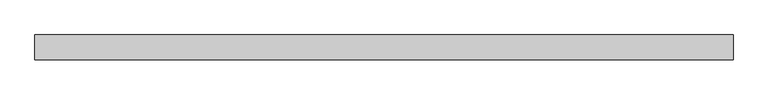
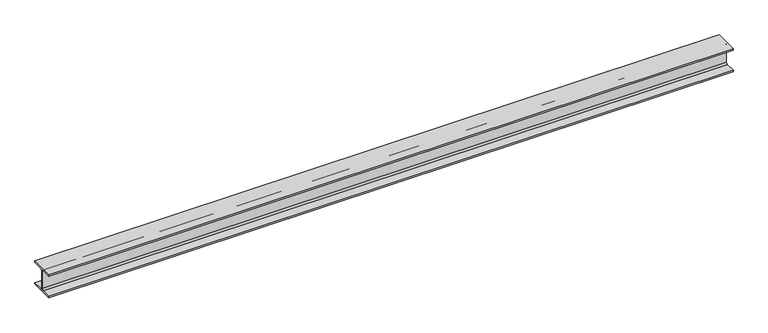
"""IFC4 building model written with IfcOpenShell, lengths in millimetres: beam geometry, 0912_Steel Framing_H-KSD3502 : H_SB_ASB_H-200x200x8x12."""

import ifcopenshell
import ifcopenshell.guid

model = None  # the IFC model being written
_history = None  # IfcOwnerHistory: only IFC2X3 demands one
_inside = {}  # id of a spatial element -> (the spatial element, [elements in it])
_under = {}  # id of a project, library or spatial element -> (it, [spatial elements below it])
_declared = {}  # id of a project -> (the project, [libraries it declares])
_typed = {}  # id of a type object -> (the type object, [elements of that type])
_made_of = {}  # id of a material, layer set ... -> (it, [elements and type objects made of it])


def new_model(schema):
    """Start an empty IFC model of exactly this schema.

    Asked for "IFC4X3", IfcOpenShell would pick the latest addendum, in which some entities
    have other attributes; the version numbers below select the first issue.
    IFC2X3 requires an IfcOwnerHistory on every rooted entity: one is made here for all.
    """
    global model, _history
    if schema == "IFC4X3":
        model = ifcopenshell.file(schema_version=(4, 3, 0, 0))
    else:
        model = ifcopenshell.file(schema=schema)
    _inside.clear()
    _under.clear()
    _declared.clear()
    _typed.clear()
    _made_of.clear()
    _history = None
    if model.schema == "IFC2X3":
        org = make("IfcOrganization", Name="unknown")
        user = make(
            "IfcPersonAndOrganization",
            ThePerson=make("IfcPerson", FamilyName="unknown"),
            TheOrganization=org,
        )
        app = make(
            "IfcApplication",
            ApplicationDeveloper=org,
            Version="unknown",
            ApplicationFullName="unknown",
            ApplicationIdentifier="unknown",
        )
        _history = make(
            "IfcOwnerHistory",
            OwningUser=user,
            OwningApplication=app,
            ChangeAction="ADDED",
            CreationDate=0,
        )
    return model


def make(cls, **values):
    """One entity of the class cls with the attributes given. An attribute that is None is left unset."""
    return model.create_entity(
        cls, **{name: value for name, value in values.items() if value is not None}
    )


def rooted(cls, **values):
    """An entity with a GlobalId (a new one), such as an element, a storey or a relation."""
    return make(cls, GlobalId=ifcopenshell.guid.new(), OwnerHistory=_history, **values)


def si_unit(unit_type, name, prefix=None):
    """IfcSIUnit, for example si_unit("LENGTHUNIT", "METRE", prefix="MILLI")."""
    return make("IfcSIUnit", UnitType=unit_type, Prefix=prefix, Name=name)


def assignment(units):
    """IfcUnitAssignment: the units of a project."""
    return None if units is None else make("IfcUnitAssignment", Units=units)


def point(xyz):
    """IfcCartesianPoint."""
    return None if xyz is None else make("IfcCartesianPoint", Coordinates=xyz)


def direction(xyz):
    """IfcDirection."""
    return None if xyz is None else make("IfcDirection", DirectionRatios=xyz)


def frame(location, z_axis=None, x_axis=None):
    """IfcAxis2Placement3D, a coordinate frame: its origin and axes. An axis left out is left unset."""
    return make(
        "IfcAxis2Placement3D",
        Location=point(location),
        Axis=direction(z_axis),
        RefDirection=direction(x_axis),
    )


def frame_2d(location, x_axis=None):
    """IfcAxis2Placement2D, a coordinate frame in the plane: its origin and x axis."""
    return make(
        "IfcAxis2Placement2D", Location=point(location), RefDirection=direction(x_axis)
    )


def origin():
    """The frame at (0, 0, 0) with its axes left unset."""
    return frame((0.0, 0.0, 0.0))


def place(relative_to, where):
    """IfcLocalPlacement: puts the frame where relative to a parent placement (None: the world)."""
    return make(
        "IfcLocalPlacement", PlacementRelTo=relative_to, RelativePlacement=where
    )


def context(
    kind, dimensions, precision=None, world=None, true_north=None, identifier=None
):
    """IfcGeometricRepresentationContext, for example the 3D "Model" context."""
    return make(
        "IfcGeometricRepresentationContext",
        ContextIdentifier=identifier,
        ContextType=kind,
        CoordinateSpaceDimension=dimensions,
        Precision=precision,
        WorldCoordinateSystem=world,
        TrueNorth=true_north,
    )


def project(units=None, contexts=None):
    """IfcProject with its units and contexts."""
    return rooted(
        "IfcProject",
        Name="project",
        RepresentationContexts=contexts,
        UnitsInContext=assignment(units),
    )


def spatial(cls, under=None, at=None, **own):
    """A site, building, storey or space (cls), placed at a placement, below another one or the project."""
    s = rooted(cls, ObjectPlacement=at, **own)
    if under is not None:
        _under.setdefault(under.id(), (under, []))[1].append(s)
    return s


def polyline(points):
    """IfcPolyline through the points."""
    return make("IfcPolyline", Points=[point(p) for p in points])


def circle_curve(where, radius):
    """IfcCircle in the frame where."""
    return make("IfcCircle", Position=where, Radius=radius)


def trimmed(basis, trim1, trim2, sense, master):
    """IfcTrimmedCurve: the piece of a basis curve between two trims."""
    return make(
        "IfcTrimmedCurve",
        BasisCurve=basis,
        Trim1=trim1,
        Trim2=trim2,
        SenseAgreement=sense,
        MasterRepresentation=master,
    )


def segment(curve, same_sense, transition):
    """IfcCompositeCurveSegment."""
    return make(
        "IfcCompositeCurveSegment",
        Transition=transition,
        SameSense=same_sense,
        ParentCurve=curve,
    )


def composite_curve(segments, self_intersect=None):
    """IfcCompositeCurve: segments joined end to end."""
    return make("IfcCompositeCurve", Segments=segments, SelfIntersect=self_intersect)


def outline(outer, holes=None, kind="AREA"):
    """IfcArbitraryClosedProfileDef: a profile drawn as a closed curve; with holes, ...WithVoids."""
    if holes is None:
        return make("IfcArbitraryClosedProfileDef", ProfileType=kind, OuterCurve=outer)
    return make(
        "IfcArbitraryProfileDefWithVoids",
        ProfileType=kind,
        OuterCurve=outer,
        InnerCurves=holes,
    )


def extrude(swept, where, along, depth):
    """IfcExtrudedAreaSolid: the profile swept, set in the frame where, extruded along a direction by depth."""
    return make(
        "IfcExtrudedAreaSolid",
        SweptArea=swept,
        Position=where,
        ExtrudedDirection=direction(along),
        Depth=depth,
    )


def shape(context_of_items, identifier, shape_type, items):
    """IfcShapeRepresentation: the items that make up one representation, for example the "Body"."""
    return make(
        "IfcShapeRepresentation",
        ContextOfItems=context_of_items,
        RepresentationIdentifier=identifier,
        RepresentationType=shape_type,
        Items=items,
    )


def source(mapping_origin, context_of_items, identifier, shape_type, items):
    """IfcRepresentationMap: a shape defined once, which mapped items show again and again."""
    return make(
        "IfcRepresentationMap",
        MappingOrigin=mapping_origin,
        MappedRepresentation=shape(context_of_items, identifier, shape_type, items),
    )


def transform(
    local_origin,
    x_axis=None,
    y_axis=None,
    z_axis=None,
    scale=None,
    scale2=None,
    scale3=None,
    uniform=True,
):
    """IfcCartesianTransformationOperator3D, or its non-uniform kind. x_axis, y_axis, z_axis: its Axis1, 2, 3."""
    if uniform:
        return make(
            "IfcCartesianTransformationOperator3D",
            Axis1=direction(x_axis),
            Axis2=direction(y_axis),
            LocalOrigin=point(local_origin),
            Scale=scale,
            Axis3=direction(z_axis),
        )
    return make(
        "IfcCartesianTransformationOperator3DnonUniform",
        Axis1=direction(x_axis),
        Axis2=direction(y_axis),
        LocalOrigin=point(local_origin),
        Scale=scale,
        Axis3=direction(z_axis),
        Scale2=scale2,
        Scale3=scale3,
    )


def mapped(mapping_source, mapping_target):
    """IfcMappedItem: shows the shape of a source again, moved by a transform."""
    return make(
        "IfcMappedItem", MappingSource=mapping_source, MappingTarget=mapping_target
    )


def made_of(thing, what):
    """Note that an element or type object is made of a material, layer set ...; save() writes the relation."""
    if what is not None:
        _made_of.setdefault(what.id(), (what, []))[1].append(thing)
    return thing


def element(
    cls,
    number,
    at=None,
    inside=None,
    cuts=None,
    type_object=None,
    material=None,
    context=None,
    identifier="Body",
    shape_type=None,
    held_by="IfcProductDefinitionShape",
    body=None,
    shapes=None,
    **own,
):
    """One element of the class cls, such as IfcWall. Its Tag is "e" and its number.

    at: its placement. inside: the storey or other place that contains it. cuts: it is an
    opening in that element (IfcRelVoidsElement). A single representation is given by context,
    identifier, shape_type and body (its items); several are given by shapes. held_by: the class
    of the entity that holds the representations. save() writes the other relations.
    """
    e = rooted(cls, Tag="e%d" % number, ObjectPlacement=at, **own)
    if body is not None:
        shapes = [shape(context, identifier, shape_type, body)]
    if shapes is not None:
        e.Representation = make(held_by, Representations=shapes)
    if inside is not None:
        _inside.setdefault(inside.id(), (inside, []))[1].append(e)
    if cuts is not None:
        rooted(
            "IfcRelVoidsElement", RelatingBuildingElement=cuts, RelatedOpeningElement=e
        )
    if type_object is not None:
        _typed.setdefault(type_object.id(), (type_object, []))[1].append(e)
    return made_of(e, material)


def aggregate(whole, parts):
    """IfcRelAggregates: a whole, such as a stair, and the parts it consists of."""
    return rooted("IfcRelAggregates", RelatingObject=whole, RelatedObjects=parts)


def save(model, path):
    """Write the relations noted so far, then the file.

    IfcRelAggregates (storeys below a building ...), IfcRelContainedInSpatialStructure (elements
    in a storey), IfcRelDefinesByType, IfcRelAssociatesMaterial and IfcRelDeclares: one each for
    every whole, place, type object, material and project.
    """
    for whole, parts in _under.values():
        aggregate(whole, parts)
    for where, things in _inside.values():
        rooted(
            "IfcRelContainedInSpatialStructure",
            RelatedElements=things,
            RelatingStructure=where,
        )
    for kind, things in _typed.values():
        rooted("IfcRelDefinesByType", RelatedObjects=things, RelatingType=kind)
    for what, things in _made_of.values():
        rooted("IfcRelAssociatesMaterial", RelatedObjects=things, RelatingMaterial=what)
    for by, libraries in _declared.values():
        rooted("IfcRelDeclares", RelatingContext=by, RelatedDefinitions=libraries)
    model.write(path)


def beam_35a77e60(model_context):
    return source(origin(), model_context, "Body", "SweptSolid", [
        extrude(outline(composite_curve([segment(polyline([(100.0, -88.0), (100.0, -100.0), (-100.0, -100.0), (-100.0, -88.0), (-17.0, -88.0)]), True, "CONTINUOUS"), segment(trimmed(circle_curve(frame_2d((-17.0, -75.0)), 13.0), [point((-17.0, -88.0))], [point((-4.0, -75.0))], True, "CARTESIAN"), True, "CONTINUOUS"), segment(polyline([(-4.0, -75.0), (-4.0, 75.0)]), True, "CONTINUOUS"), segment(trimmed(circle_curve(frame_2d((-17.0, 75.0)), 13.0), [point((-4.0, 75.0))], [point((-17.0, 88.0))], True, "CARTESIAN"), True, "CONTINUOUS"), segment(polyline([(-17.0, 88.0), (-100.0, 88.0), (-100.0, 100.0), (100.0, 100.0), (100.0, 88.0), (17.0, 88.0)]), True, "CONTINUOUS"), segment(trimmed(circle_curve(frame_2d((17.0, 75.0)), 13.0), [point((17.0, 88.0))], [point((4.0, 75.0))], True, "CARTESIAN"), True, "CONTINUOUS"), segment(polyline([(4.0, 75.0), (4.0, -75.0)]), True, "CONTINUOUS"), segment(trimmed(circle_curve(frame_2d((17.0, -75.0)), 13.0), [point((4.0, -75.0))], [point((17.0, -88.0))], True, "CARTESIAN"), True, "CONTINUOUS"), segment(polyline([(17.0, -88.0), (100.0, -88.0)]), True, "CONTINUOUS")], self_intersect=False)), frame((-2836.3595741, 0.0, 0.0), z_axis=(1.0, 0.0, 0.0), x_axis=(0.0, 1.0, 0.0)), (0.0, 0.0, 1.0), 5644.3797083),
    ])


if __name__ == "__main__":
    model = new_model("IFC4")
    model_context = context("Model", 3, world=origin())
    ifc_project = project(units=[si_unit("LENGTHUNIT", "METRE", prefix="MILLI")], contexts=[model_context])
    site = spatial("IfcSite", under=ifc_project)
    building = spatial("IfcBuilding", under=site)
    placement = place(None, origin())
    beam_shape = beam_35a77e60(model_context)
    element("IfcBeam", 1, ObjectType="0912_Steel Framing_H-KSD3502 : H_SB_ASB_H-200x200x8x12", at=placement, inside=building, context=model_context, shape_type="MappedRepresentation", body=[
        mapped(beam_shape, transform((0.0, 0.0, 0.0), x_axis=(1.0, 0.0, 0.0), y_axis=(0.0, 1.0, 0.0), z_axis=(0.0, 0.0, 1.0))),
    ])
    save(model, "model.ifc")

# Revit data of these elements
# Type "0912_Steel Framing_H-KSD3502 : H_SB_ASB_H-200x200x8x12"
#   H_WM Code_1 = "S01AA002-00001 | Main Steel Structure Fabrication Work | Shelter/Building | Medium Steel - Standard (90KG/M>Weight≥30KG/M) | Material: (   )"
#   H_WM Code_2 = "S03AA028-00001 | Main Steel Structure Erection Work | Shelter/Building | Medium Steel (90KG/M>Weight≥30KG/M) | Material: (   )"
#   H_WM Code_3 = "S01AA010-00001 | Main Steel Structure Fabrication Work | Shelter/Building | Steel Painting/Coating | for Non-Fireproofed Steel Surface, Surface Preparation, Primer, Second & Final Coat | Material: (   )"
#   H_Q'ty Cal Type Tag = "SB-Q2"
#   Width = 20.0 cm
#   Web Thickness = 0.8 cm
#   Web Fillet = 1.3 cm
#   Warping Constant = 141000.0 cm⁶
#   W = 0
#   Torsional Moment of Inertia = 26.2485 cm⁴
#   Section Area = 63.53 cm²
#   Plastic Modulus weak axis = 244.0 cm³
#   Plastic Modulus strong axis = 525.0 cm³
#   Perimeter = 1.16 m²/m
#   Nominal Weight = 49.90 kgf/m
#   Moment of Inertia weak axis = 1600.00 cm⁴
#   Moment of Inertia strong axis = 4720.00 cm⁴
#   Height = 20.0 cm
#   Flange Thickness = 1.2 cm
#   Elastic Modulus weak axis = 160.0 cm³
#   Elastic Modulus strong axis = 472.0 cm³
#   Centroid Vertical = 10.0 cm
#   Centroid Horizontal = 10.0 cm
#   Ix = 47200000
#   Length [instance default] = 1.5240 m
#   Zx = 525000
#   b = 0.2000 m
#   h = 0.2000 m
#   r = 0.0130 m
#   s = 0.0080 m
#   t = 0.0120 m
#   A = 0.006353 m²
#   Structural Material [instance default] = Steel, 45-345
#   Assembly Code = ""
# Element 1 (IfcBeam, "0912_Steel Framing_H-KSD3502 : H_SB_ASB_H-200x200x8x12")
#   Structural Material = none
# Materials
#   "Steel, 45-345": class "Metal", colour RGB 189 187 185, transparency 0, Description = "Steel 345 MPa", Cost = 0
